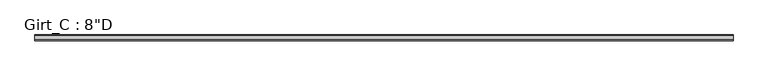
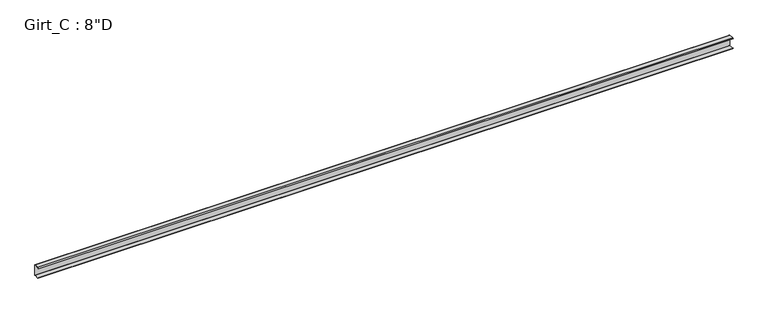
"""IFC4 building model written with IfcOpenShell, lengths in millimetres: beam geometry."""

from ifc_helpers import new_model, si_unit, point, frame, frame_2d, origin, place, context, project, spatial, polyline, circle_curve, trimmed, segment, composite_curve, outline, extrude, source, transform, mapped, element, save


def beam_3ea4ea84(model_context):
    return source(origin(), model_context, "Body", "SweptSolid", [
        extrude(outline(composite_curve([segment(polyline([(-87.5109375, 101.6), (-3.3734375, 101.6)]), True, "CONTINUOUS"), segment(trimmed(circle_curve(frame_2d((-3.3734375, 96.8375)), 4.7625), [point((-3.3734375, 101.6))], [point((1.3890625, 96.8375))], False, "CARTESIAN"), True, "CONTINUOUS"), segment(polyline([(1.3890625, 96.8375), (1.3890625, -96.8375)]), True, "CONTINUOUS"), segment(trimmed(circle_curve(frame_2d((-3.3734375, -96.8375)), 4.7625), [point((1.3890625, -96.8375))], [point((-3.3734375, -101.6))], False, "CARTESIAN"), True, "CONTINUOUS"), segment(polyline([(-3.3734375, -101.6), (-87.5109375, -101.6), (-99.7792647, -86.979177), (-97.6510975, -85.1934327), (-86.2154765, -98.821875), (-3.2694106, -98.821875)]), True, "CONTINUOUS"), segment(trimmed(circle_curve(frame_2d((-3.3748024, -96.8389339)), 1.9857399), [point((-3.2694106, -98.821875))], [point((-1.3890625, -96.8389339))], True, "CARTESIAN"), True, "CONTINUOUS"), segment(polyline([(-1.3890625, -96.8389339), (-1.3890625, 96.8381931)]), True, "CONTINUOUS"), segment(trimmed(circle_curve(frame_2d((-3.3741066, 96.8381931)), 1.9850441), [point((-1.3890625, 96.8381931))], [point((-3.3005807, 98.821875))], True, "CARTESIAN"), True, "CONTINUOUS"), segment(polyline([(-3.3005807, 98.821875), (-86.2154765, 98.821875), (-97.6278742, 85.221109), (-99.7560415, 87.0068534), (-87.5109375, 101.6)]), True, "CONTINUOUS")], self_intersect=False)), frame((-6302.375, 0.0, 0.0), z_axis=(1.0, 0.0, 0.0), x_axis=(0.0, 1.0, 0.0)), (0.0, 0.0, 1.0), 12360.275),
    ])


if __name__ == "__main__":
    model = new_model("IFC4")
    model_context = context("Model", 3, world=origin())
    ifc_project = project(units=[si_unit("LENGTHUNIT", "METRE", prefix="MILLI")], contexts=[model_context])
    site = spatial("IfcSite", under=ifc_project)
    building = spatial("IfcBuilding", under=site)
    placement = place(None, origin())
    beam_shape = beam_3ea4ea84(model_context)
    element("IfcBeam", 1, ObjectType="Girt_C : 8\"D", at=placement, inside=building, context=model_context, shape_type="MappedRepresentation", body=[
        mapped(beam_shape, transform((0.0, 0.0, 0.0), x_axis=(1.0, 0.0, 0.0), y_axis=(0.0, 1.0, 0.0), z_axis=(0.0, 0.0, 1.0))),
    ])
    save(model, "model.ifc")

# Revit data of these elements
# Type "Girt_C : 8\"D"
#   half leg = 0' - 1 3/4"
#   Web_Thickness = 0' - 0 7/64"
#   Length [instance default] = 10' - 0"
#   Leg_1 = 0' - 3 1/2"
#   Height = 0' - 8"
#   Structural Material [instance default] = none
# Element 1 (IfcBeam, "Girt_C : 8\"D")
#   Structural Material = CEE' SECTION (8.0x3.5C - SEE STRUCT. DWGS)
#   Materials on its faces: "CEE' SECTION (8.0x3.5C - SEE STRUCT. DWGS)"
# Materials
#   "CEE' SECTION (8.0x3.5C - SEE STRUCT. DWGS)": class "Metal", colour RGB 137 146 153, transparency 0, Description = "Steel, mill finish", Cost = 0
